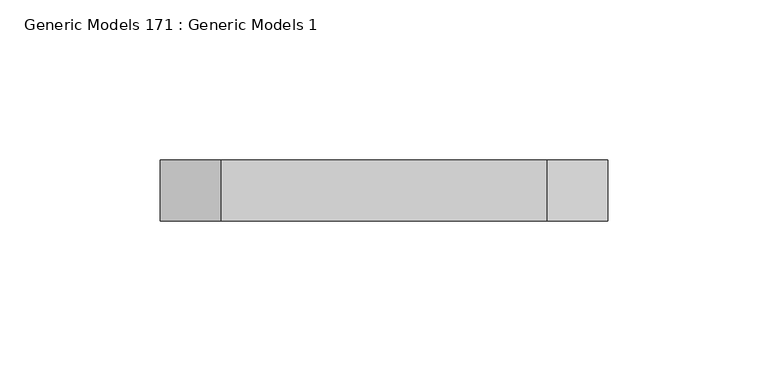
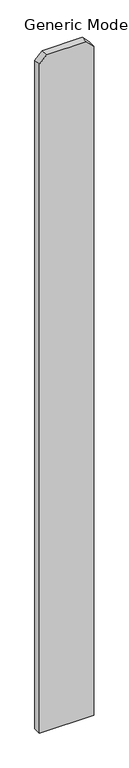
"""IFC4 building model written with IfcOpenShell, lengths in millimetres: proxy geometry, Generic Models 171 : Generic Models 1."""

import ifcopenshell
import ifcopenshell.guid

model = None  # the IFC model being written
_history = None  # IfcOwnerHistory: only IFC2X3 demands one
_inside = {}  # id of a spatial element -> (the spatial element, [elements in it])
_under = {}  # id of a project, library or spatial element -> (it, [spatial elements below it])
_declared = {}  # id of a project -> (the project, [libraries it declares])
_typed = {}  # id of a type object -> (the type object, [elements of that type])
_made_of = {}  # id of a material, layer set ... -> (it, [elements and type objects made of it])


def new_model(schema):
    """Start an empty IFC model of exactly this schema.

    Asked for "IFC4X3", IfcOpenShell would pick the latest addendum, in which some entities
    have other attributes; the version numbers below select the first issue.
    IFC2X3 requires an IfcOwnerHistory on every rooted entity: one is made here for all.
    """
    global model, _history
    if schema == "IFC4X3":
        model = ifcopenshell.file(schema_version=(4, 3, 0, 0))
    else:
        model = ifcopenshell.file(schema=schema)
    _inside.clear()
    _under.clear()
    _declared.clear()
    _typed.clear()
    _made_of.clear()
    _history = None
    if model.schema == "IFC2X3":
        org = make("IfcOrganization", Name="unknown")
        user = make(
            "IfcPersonAndOrganization",
            ThePerson=make("IfcPerson", FamilyName="unknown"),
            TheOrganization=org,
        )
        app = make(
            "IfcApplication",
            ApplicationDeveloper=org,
            Version="unknown",
            ApplicationFullName="unknown",
            ApplicationIdentifier="unknown",
        )
        _history = make(
            "IfcOwnerHistory",
            OwningUser=user,
            OwningApplication=app,
            ChangeAction="ADDED",
            CreationDate=0,
        )
    return model


def make(cls, **values):
    """One entity of the class cls with the attributes given. An attribute that is None is left unset."""
    return model.create_entity(
        cls, **{name: value for name, value in values.items() if value is not None}
    )


def rooted(cls, **values):
    """An entity with a GlobalId (a new one), such as an element, a storey or a relation."""
    return make(cls, GlobalId=ifcopenshell.guid.new(), OwnerHistory=_history, **values)


def si_unit(unit_type, name, prefix=None):
    """IfcSIUnit, for example si_unit("LENGTHUNIT", "METRE", prefix="MILLI")."""
    return make("IfcSIUnit", UnitType=unit_type, Prefix=prefix, Name=name)


def assignment(units):
    """IfcUnitAssignment: the units of a project."""
    return None if units is None else make("IfcUnitAssignment", Units=units)


def point(xyz):
    """IfcCartesianPoint."""
    return None if xyz is None else make("IfcCartesianPoint", Coordinates=xyz)


def direction(xyz):
    """IfcDirection."""
    return None if xyz is None else make("IfcDirection", DirectionRatios=xyz)


def frame(location, z_axis=None, x_axis=None):
    """IfcAxis2Placement3D, a coordinate frame: its origin and axes. An axis left out is left unset."""
    return make(
        "IfcAxis2Placement3D",
        Location=point(location),
        Axis=direction(z_axis),
        RefDirection=direction(x_axis),
    )


def origin():
    """The frame at (0, 0, 0) with its axes left unset."""
    return frame((0.0, 0.0, 0.0))


def place(relative_to, where):
    """IfcLocalPlacement: puts the frame where relative to a parent placement (None: the world)."""
    return make(
        "IfcLocalPlacement", PlacementRelTo=relative_to, RelativePlacement=where
    )


def context(
    kind, dimensions, precision=None, world=None, true_north=None, identifier=None
):
    """IfcGeometricRepresentationContext, for example the 3D "Model" context."""
    return make(
        "IfcGeometricRepresentationContext",
        ContextIdentifier=identifier,
        ContextType=kind,
        CoordinateSpaceDimension=dimensions,
        Precision=precision,
        WorldCoordinateSystem=world,
        TrueNorth=true_north,
    )


def project(units=None, contexts=None):
    """IfcProject with its units and contexts."""
    return rooted(
        "IfcProject",
        Name="project",
        RepresentationContexts=contexts,
        UnitsInContext=assignment(units),
    )


def spatial(cls, under=None, at=None, **own):
    """A site, building, storey or space (cls), placed at a placement, below another one or the project."""
    s = rooted(cls, ObjectPlacement=at, **own)
    if under is not None:
        _under.setdefault(under.id(), (under, []))[1].append(s)
    return s


def polyline(points):
    """IfcPolyline through the points."""
    return make("IfcPolyline", Points=[point(p) for p in points])


def outline(outer, holes=None, kind="AREA"):
    """IfcArbitraryClosedProfileDef: a profile drawn as a closed curve; with holes, ...WithVoids."""
    if holes is None:
        return make("IfcArbitraryClosedProfileDef", ProfileType=kind, OuterCurve=outer)
    return make(
        "IfcArbitraryProfileDefWithVoids",
        ProfileType=kind,
        OuterCurve=outer,
        InnerCurves=holes,
    )


def extrude(swept, where, along, depth):
    """IfcExtrudedAreaSolid: the profile swept, set in the frame where, extruded along a direction by depth."""
    return make(
        "IfcExtrudedAreaSolid",
        SweptArea=swept,
        Position=where,
        ExtrudedDirection=direction(along),
        Depth=depth,
    )


def shape(context_of_items, identifier, shape_type, items):
    """IfcShapeRepresentation: the items that make up one representation, for example the "Body"."""
    return make(
        "IfcShapeRepresentation",
        ContextOfItems=context_of_items,
        RepresentationIdentifier=identifier,
        RepresentationType=shape_type,
        Items=items,
    )


def source(mapping_origin, context_of_items, identifier, shape_type, items):
    """IfcRepresentationMap: a shape defined once, which mapped items show again and again."""
    return make(
        "IfcRepresentationMap",
        MappingOrigin=mapping_origin,
        MappedRepresentation=shape(context_of_items, identifier, shape_type, items),
    )


def transform(
    local_origin,
    x_axis=None,
    y_axis=None,
    z_axis=None,
    scale=None,
    scale2=None,
    scale3=None,
    uniform=True,
):
    """IfcCartesianTransformationOperator3D, or its non-uniform kind. x_axis, y_axis, z_axis: its Axis1, 2, 3."""
    if uniform:
        return make(
            "IfcCartesianTransformationOperator3D",
            Axis1=direction(x_axis),
            Axis2=direction(y_axis),
            LocalOrigin=point(local_origin),
            Scale=scale,
            Axis3=direction(z_axis),
        )
    return make(
        "IfcCartesianTransformationOperator3DnonUniform",
        Axis1=direction(x_axis),
        Axis2=direction(y_axis),
        LocalOrigin=point(local_origin),
        Scale=scale,
        Axis3=direction(z_axis),
        Scale2=scale2,
        Scale3=scale3,
    )


def mapped(mapping_source, mapping_target):
    """IfcMappedItem: shows the shape of a source again, moved by a transform."""
    return make(
        "IfcMappedItem", MappingSource=mapping_source, MappingTarget=mapping_target
    )


def made_of(thing, what):
    """Note that an element or type object is made of a material, layer set ...; save() writes the relation."""
    if what is not None:
        _made_of.setdefault(what.id(), (what, []))[1].append(thing)
    return thing


def element(
    cls,
    number,
    at=None,
    inside=None,
    cuts=None,
    type_object=None,
    material=None,
    context=None,
    identifier="Body",
    shape_type=None,
    held_by="IfcProductDefinitionShape",
    body=None,
    shapes=None,
    **own,
):
    """One element of the class cls, such as IfcWall. Its Tag is "e" and its number.

    at: its placement. inside: the storey or other place that contains it. cuts: it is an
    opening in that element (IfcRelVoidsElement). A single representation is given by context,
    identifier, shape_type and body (its items); several are given by shapes. held_by: the class
    of the entity that holds the representations. save() writes the other relations.
    """
    e = rooted(cls, Tag="e%d" % number, ObjectPlacement=at, **own)
    if body is not None:
        shapes = [shape(context, identifier, shape_type, body)]
    if shapes is not None:
        e.Representation = make(held_by, Representations=shapes)
    if inside is not None:
        _inside.setdefault(inside.id(), (inside, []))[1].append(e)
    if cuts is not None:
        rooted(
            "IfcRelVoidsElement", RelatingBuildingElement=cuts, RelatedOpeningElement=e
        )
    if type_object is not None:
        _typed.setdefault(type_object.id(), (type_object, []))[1].append(e)
    return made_of(e, material)


def aggregate(whole, parts):
    """IfcRelAggregates: a whole, such as a stair, and the parts it consists of."""
    return rooted("IfcRelAggregates", RelatingObject=whole, RelatedObjects=parts)


def save(model, path):
    """Write the relations noted so far, then the file.

    IfcRelAggregates (storeys below a building ...), IfcRelContainedInSpatialStructure (elements
    in a storey), IfcRelDefinesByType, IfcRelAssociatesMaterial and IfcRelDeclares: one each for
    every whole, place, type object, material and project.
    """
    for whole, parts in _under.values():
        aggregate(whole, parts)
    for where, things in _inside.values():
        rooted(
            "IfcRelContainedInSpatialStructure",
            RelatedElements=things,
            RelatingStructure=where,
        )
    for kind, things in _typed.values():
        rooted("IfcRelDefinesByType", RelatedObjects=things, RelatingType=kind)
    for what, things in _made_of.values():
        rooted("IfcRelAssociatesMaterial", RelatedObjects=things, RelatingMaterial=what)
    for by, libraries in _declared.values():
        rooted("IfcRelDeclares", RelatingContext=by, RelatedDefinitions=libraries)
    model.write(path)


def generic_models_171_generic_models_1_1e9a53e4(model_context):
    return source(origin(), model_context, "Body", "SweptSolid", [
        extrude(outline(polyline([(76.2, 56056.2125), (1885.95, 56056.2125), (1905.0, 56037.1625), (1905.0, 55935.5625), (1885.95, 55916.5125), (76.2, 55916.5125), (76.2, 56056.2125)])), frame((0.0, 547.6875, 0.0), z_axis=(0.0, 1.0, 0.0), x_axis=(0.0, 0.0, 1.0)), (0.0, 0.0, 1.0), 19.05),
    ])


if __name__ == "__main__":
    model = new_model("IFC4")
    model_context = context("Model", 3, world=origin())
    ifc_project = project(units=[si_unit("LENGTHUNIT", "METRE", prefix="MILLI")], contexts=[model_context])
    site = spatial("IfcSite", under=ifc_project)
    building = spatial("IfcBuilding", under=site)
    placement = place(None, origin())
    generic_models_171_generic_models_1_shape = generic_models_171_generic_models_1_1e9a53e4(model_context)
    element("IfcBuildingElementProxy", 1, Name="Generic Models 171 : Generic Models 1", ObjectType="Generic Models 171 : Generic Models 1", at=placement, inside=building, context=model_context, shape_type="MappedRepresentation", body=[
        mapped(generic_models_171_generic_models_1_shape, transform((0.0, 0.0, 0.0), x_axis=(1.0, 0.0, 0.0), y_axis=(0.0, 1.0, 0.0), z_axis=(0.0, 0.0, 1.0))),
    ])
    save(model, "model.ifc")

# Revit data of these elements
# Element 1 (IfcBuildingElementProxy, "Generic Models 171 : Generic Models 1")
#   Materials on its faces: "VERTICAL 1X6 CEDAR PLANKS W/ CLEAR WOOD SEALER"
# Materials
#   "VERTICAL 1X6 CEDAR PLANKS W/ CLEAR WOOD SEALER": class "Wood", colour RGB 234 198 147, transparency 0, Description = "Pinus Echinata", Cost = 0
